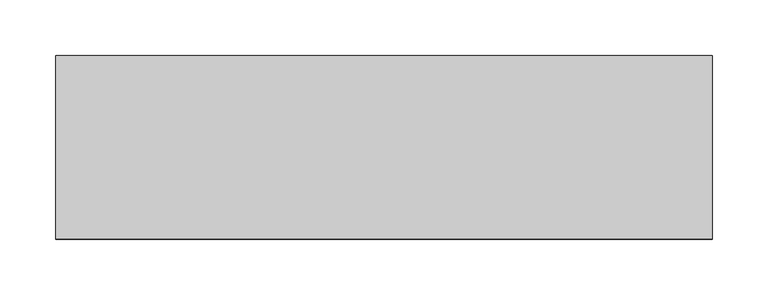
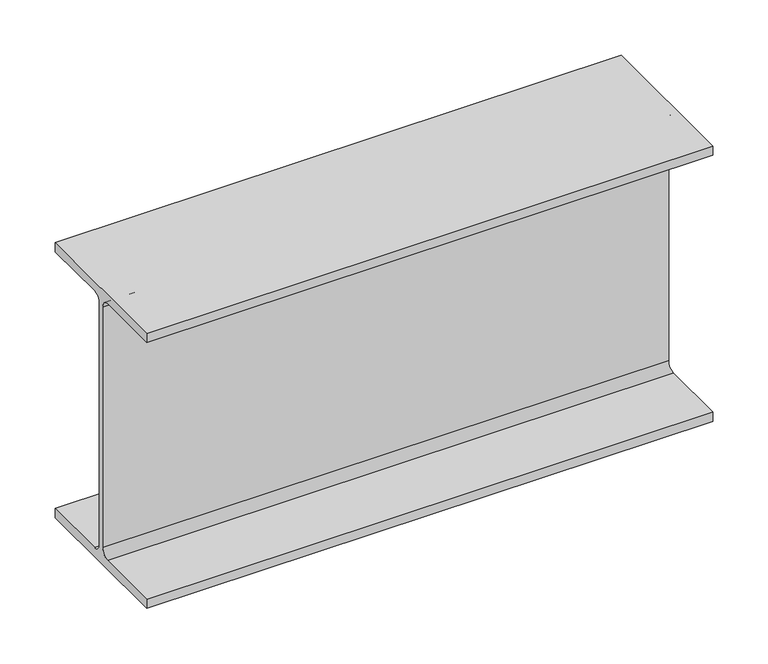
"""IFC4 building model written with IfcOpenShell, lengths in millimetres: beam geometry, Old_Steel Beam_H-KSD3502 : H_SB_ASB_H-300×150x6.5x9."""

from ifc_helpers import new_model, si_unit, point, frame, frame_2d, origin, place, context, project, spatial, polyline, circle_curve, trimmed, segment, composite_curve, outline, extrude, source, transform, mapped, element, save


def beam_5c238520(model_context):
    return source(origin(), model_context, "Body", "SweptSolid", [
        extrude(outline(composite_curve([segment(polyline([(82.5, -141.5), (82.5, -151.7), (-82.5, -151.7), (-82.5, -141.5), (-11.9, -141.5)]), True, "CONTINUOUS"), segment(trimmed(circle_curve(frame_2d((-11.9, -132.6)), 8.9), [point((-11.9, -141.5))], [point((-3.0, -132.6))], True, "CARTESIAN"), True, "CONTINUOUS"), segment(polyline([(-3.0, -132.6), (-3.0, 132.6)]), True, "CONTINUOUS"), segment(trimmed(circle_curve(frame_2d((-11.9, 132.6)), 8.9), [point((-3.0, 132.6))], [point((-11.9, 141.5))], True, "CARTESIAN"), True, "CONTINUOUS"), segment(polyline([(-11.9, 141.5), (-82.5, 141.5), (-82.5, 151.7), (82.5, 151.7), (82.5, 141.5), (11.9, 141.5)]), True, "CONTINUOUS"), segment(trimmed(circle_curve(frame_2d((11.9, 132.6)), 8.9), [point((11.9, 141.5))], [point((3.0, 132.6))], True, "CARTESIAN"), True, "CONTINUOUS"), segment(polyline([(3.0, 132.6), (3.0, -132.6)]), True, "CONTINUOUS"), segment(trimmed(circle_curve(frame_2d((11.9, -132.6)), 8.9), [point((3.0, -132.6))], [point((11.9, -141.5))], True, "CARTESIAN"), True, "CONTINUOUS"), segment(polyline([(11.9, -141.5), (82.5, -141.5)]), True, "CONTINUOUS")], self_intersect=False)), frame((-282.3, 0.0, 0.0), z_axis=(1.0, 0.0, 0.0), x_axis=(0.0, 1.0, 0.0)), (0.0, 0.0, 1.0), 589.6),
    ])


if __name__ == "__main__":
    model = new_model("IFC4")
    model_context = context("Model", 3, world=origin())
    ifc_project = project(units=[si_unit("LENGTHUNIT", "METRE", prefix="MILLI")], contexts=[model_context])
    site = spatial("IfcSite", under=ifc_project)
    building = spatial("IfcBuilding", under=site)
    placement = place(None, origin())
    beam_shape = beam_5c238520(model_context)
    element("IfcBeam", 1, ObjectType="Old_Steel Beam_H-KSD3502 : H_SB_ASB_H-300×150x6.5x9", at=placement, inside=building, context=model_context, shape_type="MappedRepresentation", body=[
        mapped(beam_shape, transform((0.0, 0.0, 0.0), x_axis=(1.0, 0.0, 0.0), y_axis=(0.0, 1.0, 0.0), z_axis=(0.0, 0.0, 1.0))),
    ])
    save(model, "model.ifc")

# Revit data of these elements
# Type "Old_Steel Beam_H-KSD3502 : H_SB_ASB_H-300×150x6.5x9"
#   Width = 15.0 cm
#   Web Thickness = 0.65 cm
#   Web Fillet = 1.3 cm
#   Warping Constant = 107174.0 cm⁶
#   Torsional Moment of Inertia = 9.9539 cm⁴
#   Torsional Modulus = 1.0 cm³
#   Section Area = 46.78 cm²
#   Plastic Modulus weak axis = 105.0 cm³
#   Plastic Modulus strong axis = 542.0 cm³
#   Perimeter = 1.17 m²/m
#   Nominal Weight = 36.70 kgf/m
#   Moment of Inertia weak axis = 508.00 cm⁴
#   Moment of Inertia strong axis = 7210.00 cm⁴
#   Height = 30.0 cm
#   Flange Thickness = 0.9 cm
#   Elastic Modulus weak axis = 67.7 cm³
#   Elastic Modulus strong axis = 481.0 cm³
#   Centroid Vertical = 15.0 cm
#   Centroid Horizontal = 7.5 cm
#   Length [instance default] = 1.5240 m
#   Structural Material [instance default] = Steel, 45-345
#   Assembly Code = ""
# Element 1 (IfcBeam, "Old_Steel Beam_H-KSD3502 : H_SB_ASB_H-300×150x6.5x9")
#   Structural Material = none
# Materials
#   "Steel, 45-345": class "Metal", colour RGB 189 187 185, transparency 0, Description = "Steel 345 MPa", Cost = 0
